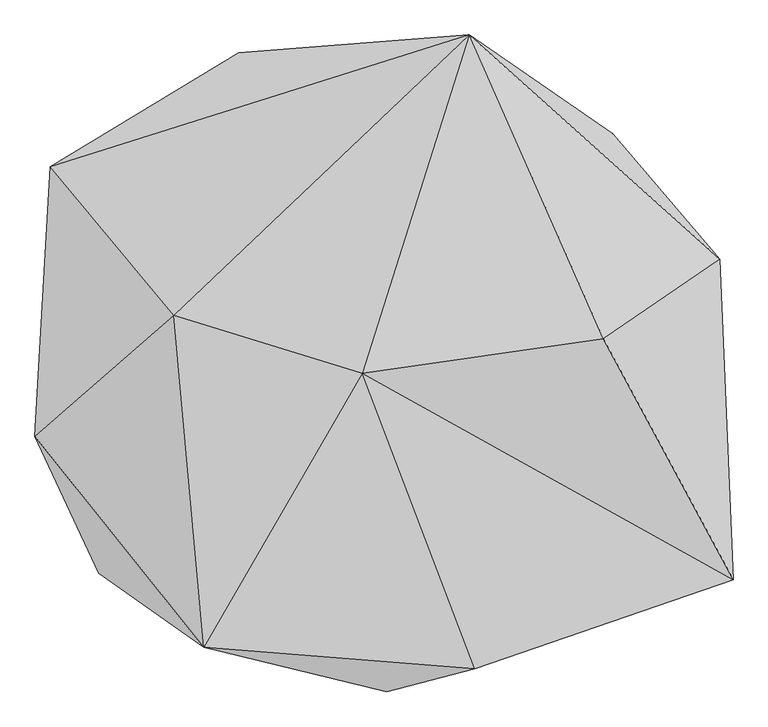
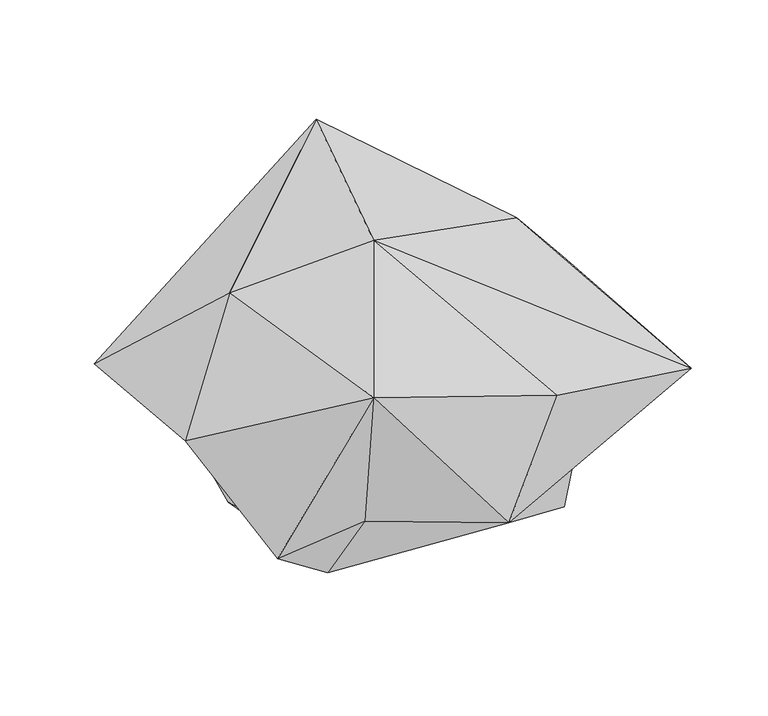
"""IFC4 building model written with IfcOpenShell, lengths in millimetres: geographic element geometry, Enscape AssetDefinition - Bush 080 Festuca Sunrise : Enscape AssetDefinition - Bush 080 Festuca Sunrise."""

from ifc_helpers import new_model, si_unit, origin, place, context, project, spatial, faceted_brep, source, transform, mapped, element, save


def geographic_element_8bdaba8b(model_context):
    return source(origin(), model_context, "Body", "Brep", [
        faceted_brep([(373.6900091, 368.9709902, 97.3739997), (336.9539976, 97.5830033, 185.6140047), (393.8780129, -13.8940001, 41.3549989), (322.2149909, -271.9359994, 172.8730053), (562.2000098, -329.9309909, 302.4179935), (541.5340066, 172.4160016, 290.989995), (296.77701, -257.5939894, -3.0759999), (206.6870034, 193.095997, -4.0679998), (92.2999978, 378.2980144, 69.2259967), (148.6970037, 523.8050222, 564.981997), (358.6530089, 47.4120006, 528.7659764), (-212.2880071, 496.0350096, 250.3220141), (-313.9789999, 84.9940032, 550.1919985), (-507.776022, 317.2590137, 295.4779863), (-18.4870008, -6.6530001, 636.1600161), (-267.0510113, -435.8809888, 580.648005), (157.6900035, -469.4710076, 459.0910077), (-531.637013, -105.0139964, 363.4609878), (-376.4280081, 187.8540069, 192.1650022), (-227.0220071, 274.6909857, 37.9679985), (-431.6860139, -319.6119964, 156.1020017), (-319.5909858, 81.4630017, 18.4579995), (-367.2449887, -70.3610033, 103.8990021), (-265.2989924, -241.6770011, 15.7529991), (-222.5389928, -322.3780096, 180.4720014), (-119.8190004, 257.871002, -7.4499999), (19.5269994, -505.0989985, 202.8889954)], [[[0, 1, 2]], [[1, 3, 2]], [[4, 3, 1]], [[1, 0, 5]], [[4, 1, 5]], [[2, 3, 6]], [[2, 6, 7]], [[2, 7, 0]], [[8, 0, 7]], [[8, 9, 0]], [[9, 5, 0]], [[4, 5, 10]], [[9, 10, 5]], [[11, 9, 8]], [[12, 9, 13]], [[14, 9, 12]], [[14, 10, 9]], [[13, 9, 11]], [[14, 4, 10]], [[12, 15, 14]], [[16, 4, 14]], [[15, 16, 14]], [[12, 13, 17]], [[12, 17, 15]], [[17, 13, 18]], [[18, 13, 11]], [[11, 19, 18]], [[8, 19, 11]], [[17, 18, 20]], [[18, 21, 22]], [[19, 21, 18]], [[18, 22, 20]], [[20, 15, 17]], [[22, 23, 20]], [[24, 20, 23]], [[20, 24, 15]], [[22, 21, 23]], [[19, 25, 21]], [[21, 25, 6]], [[23, 21, 6]], [[19, 8, 25]], [[25, 8, 7]], [[7, 6, 25]], [[3, 26, 6]], [[6, 26, 23]], [[26, 24, 23]], [[24, 26, 15]], [[26, 3, 4]], [[16, 26, 4]], [[16, 15, 26]]]),
    ])


if __name__ == "__main__":
    model = new_model("IFC4")
    model_context = context("Model", 3, world=origin())
    ifc_project = project(units=[si_unit("LENGTHUNIT", "METRE", prefix="MILLI")], contexts=[model_context])
    site = spatial("IfcSite", under=ifc_project)
    building = spatial("IfcBuilding", under=site)
    placement = place(None, origin())
    geographic_element_shape = geographic_element_8bdaba8b(model_context)
    element("IfcGeographicElement", 1, ObjectType="Enscape AssetDefinition - Bush 080 Festuca Sunrise : Enscape AssetDefinition - Bush 080 Festuca Sunrise", at=placement, inside=building, context=model_context, shape_type="MappedRepresentation", body=[
        mapped(geographic_element_shape, transform((0.0, 0.0, 0.0), x_axis=(1.0, 0.0, 0.0), y_axis=(0.0, 1.0, 0.0), z_axis=(0.0, 0.0, 1.0))),
    ])
    save(model, "model.ifc")

# Revit data of these elements
# Type "Enscape AssetDefinition - Bush 080 Festuca Sunrise : Enscape AssetDefinition - Bush 080 Festuca Sunrise"
#   EnscapeAssetSource = "REMOTE"
#   EnscapeAssetId = "7b807a01-288a-48fd-b4bd-fa406d690ed4"
#   Height = 0.63616 m
#   EnscapeNativeAssetHeight = 0.63616 m
#   Default Elevation = 0
